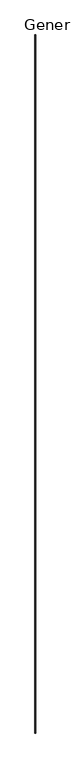
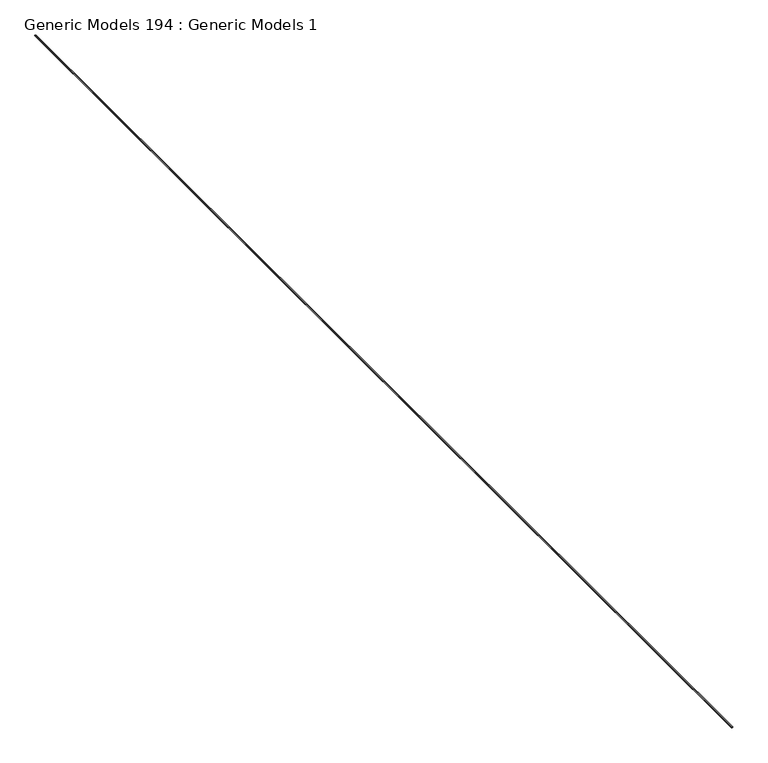
"""IFC4 building model written with IfcOpenShell, lengths in millimetres: proxy geometry, Generic Models 194 : Generic Models 1."""

import ifcopenshell
import ifcopenshell.guid

model = None  # the IFC model being written
_history = None  # IfcOwnerHistory: only IFC2X3 demands one
_inside = {}  # id of a spatial element -> (the spatial element, [elements in it])
_under = {}  # id of a project, library or spatial element -> (it, [spatial elements below it])
_declared = {}  # id of a project -> (the project, [libraries it declares])
_typed = {}  # id of a type object -> (the type object, [elements of that type])
_made_of = {}  # id of a material, layer set ... -> (it, [elements and type objects made of it])


def new_model(schema):
    """Start an empty IFC model of exactly this schema.

    Asked for "IFC4X3", IfcOpenShell would pick the latest addendum, in which some entities
    have other attributes; the version numbers below select the first issue.
    IFC2X3 requires an IfcOwnerHistory on every rooted entity: one is made here for all.
    """
    global model, _history
    if schema == "IFC4X3":
        model = ifcopenshell.file(schema_version=(4, 3, 0, 0))
    else:
        model = ifcopenshell.file(schema=schema)
    _inside.clear()
    _under.clear()
    _declared.clear()
    _typed.clear()
    _made_of.clear()
    _history = None
    if model.schema == "IFC2X3":
        org = make("IfcOrganization", Name="unknown")
        user = make(
            "IfcPersonAndOrganization",
            ThePerson=make("IfcPerson", FamilyName="unknown"),
            TheOrganization=org,
        )
        app = make(
            "IfcApplication",
            ApplicationDeveloper=org,
            Version="unknown",
            ApplicationFullName="unknown",
            ApplicationIdentifier="unknown",
        )
        _history = make(
            "IfcOwnerHistory",
            OwningUser=user,
            OwningApplication=app,
            ChangeAction="ADDED",
            CreationDate=0,
        )
    return model


def make(cls, **values):
    """One entity of the class cls with the attributes given. An attribute that is None is left unset."""
    return model.create_entity(
        cls, **{name: value for name, value in values.items() if value is not None}
    )


def rooted(cls, **values):
    """An entity with a GlobalId (a new one), such as an element, a storey or a relation."""
    return make(cls, GlobalId=ifcopenshell.guid.new(), OwnerHistory=_history, **values)


def si_unit(unit_type, name, prefix=None):
    """IfcSIUnit, for example si_unit("LENGTHUNIT", "METRE", prefix="MILLI")."""
    return make("IfcSIUnit", UnitType=unit_type, Prefix=prefix, Name=name)


def assignment(units):
    """IfcUnitAssignment: the units of a project."""
    return None if units is None else make("IfcUnitAssignment", Units=units)


def point(xyz):
    """IfcCartesianPoint."""
    return None if xyz is None else make("IfcCartesianPoint", Coordinates=xyz)


def direction(xyz):
    """IfcDirection."""
    return None if xyz is None else make("IfcDirection", DirectionRatios=xyz)


def frame(location, z_axis=None, x_axis=None):
    """IfcAxis2Placement3D, a coordinate frame: its origin and axes. An axis left out is left unset."""
    return make(
        "IfcAxis2Placement3D",
        Location=point(location),
        Axis=direction(z_axis),
        RefDirection=direction(x_axis),
    )


def origin():
    """The frame at (0, 0, 0) with its axes left unset."""
    return frame((0.0, 0.0, 0.0))


def place(relative_to, where):
    """IfcLocalPlacement: puts the frame where relative to a parent placement (None: the world)."""
    return make(
        "IfcLocalPlacement", PlacementRelTo=relative_to, RelativePlacement=where
    )


def context(
    kind, dimensions, precision=None, world=None, true_north=None, identifier=None
):
    """IfcGeometricRepresentationContext, for example the 3D "Model" context."""
    return make(
        "IfcGeometricRepresentationContext",
        ContextIdentifier=identifier,
        ContextType=kind,
        CoordinateSpaceDimension=dimensions,
        Precision=precision,
        WorldCoordinateSystem=world,
        TrueNorth=true_north,
    )


def project(units=None, contexts=None):
    """IfcProject with its units and contexts."""
    return rooted(
        "IfcProject",
        Name="project",
        RepresentationContexts=contexts,
        UnitsInContext=assignment(units),
    )


def spatial(cls, under=None, at=None, **own):
    """A site, building, storey or space (cls), placed at a placement, below another one or the project."""
    s = rooted(cls, ObjectPlacement=at, **own)
    if under is not None:
        _under.setdefault(under.id(), (under, []))[1].append(s)
    return s


def polyline(points):
    """IfcPolyline through the points."""
    return make("IfcPolyline", Points=[point(p) for p in points])


def circle_curve(where, radius):
    """IfcCircle in the frame where."""
    return make("IfcCircle", Position=where, Radius=radius)


def ellipse_curve(where, semi_axis1, semi_axis2):
    """IfcEllipse in the frame where."""
    return make(
        "IfcEllipse", Position=where, SemiAxis1=semi_axis1, SemiAxis2=semi_axis2
    )


def trimmed(basis, trim1, trim2, sense, master):
    """IfcTrimmedCurve: the piece of a basis curve between two trims."""
    return make(
        "IfcTrimmedCurve",
        BasisCurve=basis,
        Trim1=trim1,
        Trim2=trim2,
        SenseAgreement=sense,
        MasterRepresentation=master,
    )


def shape(context_of_items, identifier, shape_type, items):
    """IfcShapeRepresentation: the items that make up one representation, for example the "Body"."""
    return make(
        "IfcShapeRepresentation",
        ContextOfItems=context_of_items,
        RepresentationIdentifier=identifier,
        RepresentationType=shape_type,
        Items=items,
    )


def source(mapping_origin, context_of_items, identifier, shape_type, items):
    """IfcRepresentationMap: a shape defined once, which mapped items show again and again."""
    return make(
        "IfcRepresentationMap",
        MappingOrigin=mapping_origin,
        MappedRepresentation=shape(context_of_items, identifier, shape_type, items),
    )


def transform(
    local_origin,
    x_axis=None,
    y_axis=None,
    z_axis=None,
    scale=None,
    scale2=None,
    scale3=None,
    uniform=True,
):
    """IfcCartesianTransformationOperator3D, or its non-uniform kind. x_axis, y_axis, z_axis: its Axis1, 2, 3."""
    if uniform:
        return make(
            "IfcCartesianTransformationOperator3D",
            Axis1=direction(x_axis),
            Axis2=direction(y_axis),
            LocalOrigin=point(local_origin),
            Scale=scale,
            Axis3=direction(z_axis),
        )
    return make(
        "IfcCartesianTransformationOperator3DnonUniform",
        Axis1=direction(x_axis),
        Axis2=direction(y_axis),
        LocalOrigin=point(local_origin),
        Scale=scale,
        Axis3=direction(z_axis),
        Scale2=scale2,
        Scale3=scale3,
    )


def mapped(mapping_source, mapping_target):
    """IfcMappedItem: shows the shape of a source again, moved by a transform."""
    return make(
        "IfcMappedItem", MappingSource=mapping_source, MappingTarget=mapping_target
    )


def made_of(thing, what):
    """Note that an element or type object is made of a material, layer set ...; save() writes the relation."""
    if what is not None:
        _made_of.setdefault(what.id(), (what, []))[1].append(thing)
    return thing


def element(
    cls,
    number,
    at=None,
    inside=None,
    cuts=None,
    type_object=None,
    material=None,
    context=None,
    identifier="Body",
    shape_type=None,
    held_by="IfcProductDefinitionShape",
    body=None,
    shapes=None,
    **own,
):
    """One element of the class cls, such as IfcWall. Its Tag is "e" and its number.

    at: its placement. inside: the storey or other place that contains it. cuts: it is an
    opening in that element (IfcRelVoidsElement). A single representation is given by context,
    identifier, shape_type and body (its items); several are given by shapes. held_by: the class
    of the entity that holds the representations. save() writes the other relations.
    """
    e = rooted(cls, Tag="e%d" % number, ObjectPlacement=at, **own)
    if body is not None:
        shapes = [shape(context, identifier, shape_type, body)]
    if shapes is not None:
        e.Representation = make(held_by, Representations=shapes)
    if inside is not None:
        _inside.setdefault(inside.id(), (inside, []))[1].append(e)
    if cuts is not None:
        rooted(
            "IfcRelVoidsElement", RelatingBuildingElement=cuts, RelatedOpeningElement=e
        )
    if type_object is not None:
        _typed.setdefault(type_object.id(), (type_object, []))[1].append(e)
    return made_of(e, material)


def aggregate(whole, parts):
    """IfcRelAggregates: a whole, such as a stair, and the parts it consists of."""
    return rooted("IfcRelAggregates", RelatingObject=whole, RelatedObjects=parts)


def save(model, path):
    """Write the relations noted so far, then the file.

    IfcRelAggregates (storeys below a building ...), IfcRelContainedInSpatialStructure (elements
    in a storey), IfcRelDefinesByType, IfcRelAssociatesMaterial and IfcRelDeclares: one each for
    every whole, place, type object, material and project.
    """
    for whole, parts in _under.values():
        aggregate(whole, parts)
    for where, things in _inside.values():
        rooted(
            "IfcRelContainedInSpatialStructure",
            RelatedElements=things,
            RelatingStructure=where,
        )
    for kind, things in _typed.values():
        rooted("IfcRelDefinesByType", RelatedObjects=things, RelatingType=kind)
    for what, things in _made_of.values():
        rooted("IfcRelAssociatesMaterial", RelatedObjects=things, RelatingMaterial=what)
    for by, libraries in _declared.values():
        rooted("IfcRelDeclares", RelatingContext=by, RelatedDefinitions=libraries)
    model.write(path)


def plane_surface(at):
    """IfcPlane: the flat surface through the origin of the frame at, square to its z axis."""
    return make("IfcPlane", Position=at)


def cylinder_surface(at, radius):
    """IfcCylindricalSurface: all points at the distance radius from the z axis of the frame at."""
    return make("IfcCylindricalSurface", Position=at, Radius=radius)


def revolved_surface(curve, axis_point, axis_direction):
    """IfcSurfaceOfRevolution: the curve turned about the line through axis_point along axis_direction."""
    return make(
        "IfcSurfaceOfRevolution",
        SweptCurve=make("IfcArbitraryOpenProfileDef", ProfileType="CURVE", Curve=curve),
        AxisPosition=make("IfcAxis1Placement", Location=point(axis_point), Axis=direction(axis_direction)),
    )


def extruded_surface(curve, direction_of_extrusion, depth):
    """IfcSurfaceOfLinearExtrusion: the curve pushed along a direction by depth."""
    return make(
        "IfcSurfaceOfLinearExtrusion",
        SweptCurve=make("IfcArbitraryOpenProfileDef", ProfileType="CURVE", Curve=curve),
        ExtrudedDirection=direction(direction_of_extrusion),
        Depth=depth,
    )


def advanced_brep(points, edges, surfaces, faces):
    """IfcAdvancedBrep: a solid bounded by faces that lie on surfaces and meet in shared edges.

    An edge is (start, end): straight between two places in points (the first is 0);
    or (start, end, curve); or (start, end, curve, False) where it runs against its curve.
    A face is (place in surfaces, loops), or (place, loops, False) where it looks against
    its surface's normal. A loop lists edges by number (the first is 1), with a minus sign
    where the edge is run from its end to its start. The first loop is the outer one.
    """
    corners = [point(p) for p in points]
    vertices = [make("IfcVertexPoint", VertexGeometry=c) for c in corners]
    made = []
    for start, end, *more in edges:
        made.append(
            make(
                "IfcEdgeCurve",
                EdgeStart=vertices[start],
                EdgeEnd=vertices[end],
                EdgeGeometry=more[0] if more else make("IfcPolyline", Points=[corners[start], corners[end]]),
                SameSense=more[1] if len(more) > 1 else True,
            )
        )
    hull = []
    for where, loops, *sense in faces:
        bounds = []
        for j, loop in enumerate(loops):
            ring = [make("IfcOrientedEdge", EdgeElement=made[abs(k) - 1], Orientation=k > 0) for k in loop]
            bounds.append(
                make(
                    "IfcFaceOuterBound" if j == 0 else "IfcFaceBound",
                    Bound=make("IfcEdgeLoop", EdgeList=ring),
                    Orientation=True,
                )
            )
        hull.append(make("IfcAdvancedFace", Bounds=bounds, FaceSurface=surfaces[where], SameSense=sense[0] if sense else True))
    return make("IfcAdvancedBrep", Outer=make("IfcClosedShell", CfsFaces=hull))


def generic_models_194_generic_models_1_cef9da7c(model_context):
    return source(origin(), model_context, "Body", "AdvancedBrep", [
        advanced_brep(
        [(-6651.2562339, 11981.8769662, 126151.8372608), (-6651.2562339, 11981.8769662, 126161.3622608), (-6646.4937339, 11981.8769662, 126161.3622608), (-6645.0660949, 11981.8769662, 126159.456273), (-6645.0660949, 11981.8769662, 126153.7432487), (-6646.4937339, 11981.8769662, 126151.8372608), (-6651.2562339, -7068.1230338, 126151.8372608), (-6646.4937339, -7068.1230338, 126151.8372608), (-6645.0660949, -7068.1230338, 126153.7432487), (-6645.0660949, -7068.1230338, 126159.456273), (-6646.4937339, -7068.1230338, 126161.3622608), (-6651.2562339, -7068.1230338, 126161.3622608)],
        [
            (0, 1, circle_curve(frame((-6655.6283446, 11981.8769662, 126156.5997608), z_axis=(0.0, -1.0, 0.0), x_axis=(0.0, 0.0, -1.0)), 6.4650413)),
            (1, 2),
            (2, 3, circle_curve(frame((-6650.8658446, 11981.8769662, 126156.5997608), z_axis=(0.0, 1.0, 0.0), x_axis=(0.0, 0.0, -1.0)), 6.4650413)),
            (3, 4, ellipse_curve(frame((-6639.3499839, 11981.8769662, 126156.5997608), z_axis=(0.0, 1.0, 0.0), x_axis=(-1.0, 0.0, 0.0)), 7.14375, 4.7625)),
            (4, 5, circle_curve(frame((-6650.8658446, 11981.8769662, 126156.5997608), z_axis=(0.0, 1.0, 0.0), x_axis=(0.0, 0.0, -1.0)), 6.4650413)),
            (5, 0),
            (6, 7),
            (7, 8, circle_curve(frame((-6650.8658446, -7068.1230338, 126156.5997608), z_axis=(0.0, -1.0, 0.0), x_axis=(0.0, 0.0, -1.0)), 6.4650413)),
            (8, 9, ellipse_curve(frame((-6639.3499839, -7068.1230338, 126156.5997608), z_axis=(0.0, -1.0, 0.0), x_axis=(-1.0, 0.0, 0.0)), 7.14375, 4.7625)),
            (9, 10, circle_curve(frame((-6650.8658446, -7068.1230338, 126156.5997608), z_axis=(0.0, -1.0, 0.0), x_axis=(0.0, 0.0, -1.0)), 6.4650413)),
            (10, 11),
            (11, 6, circle_curve(frame((-6655.6283446, -7068.1230338, 126156.5997608), z_axis=(0.0, 1.0, 0.0), x_axis=(0.0, 0.0, -1.0)), 6.4650413)),
            (3, 9),
            (8, 4),
            (0, 6),
            (11, 1),
            (10, 2),
            (7, 5),
        ],
        [
            plane_surface(frame((-6651.2562339, 11981.8769662, 126161.3622608), z_axis=(0.0, 1.0, 0.0), x_axis=(-1.0, 0.0, 0.0))),
            plane_surface(frame((-6651.2562339, -7068.1230338, 126161.3622608), z_axis=(0.0, -1.0, 0.0), x_axis=(-1.0, 0.0, 0.0))),
            extruded_surface(trimmed(ellipse_curve(frame((-6639.3499839, -7068.1230338, 126156.5997608), z_axis=(0.0, 1.0, 0.0), x_axis=(-1.0, 0.0, 0.0)), 7.14375, 4.7625), [point((-6645.0660949, -7068.1230338, 126159.456273))], [point((-6645.0660949, -7068.1230338, 126153.7432487))], True, "CARTESIAN"), (0.0, 19050.0, 0.0), 19050.0),
            revolved_surface(polyline([(-6655.6283446, -7068.1230338000005, 126150.1347195), (-6655.6283446, 11981.8769662, 126150.1347195)]), (-6655.6283446, 11981.8769662, 126156.5997608), (0.0, -1.0, 0.0)),
            plane_surface(frame((-6651.2562339, 11981.8769662, 126161.3622608), z_axis=(0.0, 0.0, 1.0), x_axis=(0.0, -1.0, 0.0))),
            cylinder_surface(frame((-6650.8658446, 11981.8769662, 126156.5997608), z_axis=(0.0, 1.0, 0.0), x_axis=(0.0, 0.0, -1.0)), 6.4650413),
            plane_surface(frame((-6646.4937339, 11981.8769662, 126151.8372608), z_axis=(0.0, 0.0, -1.0), x_axis=(0.0, -1.0, 0.0))),
        ],
        [
            (0, [[1, 2, 3, 4, 5, 6]]),
            (1, [[7, 8, 9, 10, 11, 12]]),
            (2, [[-4, 13, -9, 14]]),
            (3, [[-1, 15, -12, 16]]),
            (4, [[-2, -16, -11, 17]]),
            (5, [[-3, -17, -10, -13]]),
            (5, [[-5, -14, -8, 18]]),
            (6, [[-6, -18, -7, -15]]),
        ],
    ),
    ])


if __name__ == "__main__":
    model = new_model("IFC4")
    model_context = context("Model", 3, world=origin())
    ifc_project = project(units=[si_unit("LENGTHUNIT", "METRE", prefix="MILLI")], contexts=[model_context])
    site = spatial("IfcSite", under=ifc_project)
    building = spatial("IfcBuilding", under=site)
    placement = place(None, origin())
    generic_models_194_generic_models_1_shape = generic_models_194_generic_models_1_cef9da7c(model_context)
    element("IfcBuildingElementProxy", 1, Name="Generic Models 194 : Generic Models 1", ObjectType="Generic Models 194 : Generic Models 1", at=placement, inside=building, context=model_context, shape_type="MappedRepresentation", body=[
        mapped(generic_models_194_generic_models_1_shape, transform((0.0, 0.0, 0.0), x_axis=(1.0, 0.0, 0.0), y_axis=(0.0, 1.0, 0.0), z_axis=(0.0, 0.0, 1.0))),
    ])
    save(model, "model.ifc")

# Revit data of these elements
# Element 1 (IfcBuildingElementProxy, "Generic Models 194 : Generic Models 1")
#   Materials on its faces: "_SEALANT AND BACKROD, IF NEC."
# Materials
#   "_SEALANT AND BACKROD, IF NEC.": class "Generic", colour RGB 190 220 196, transparency 0, Cost = 0
